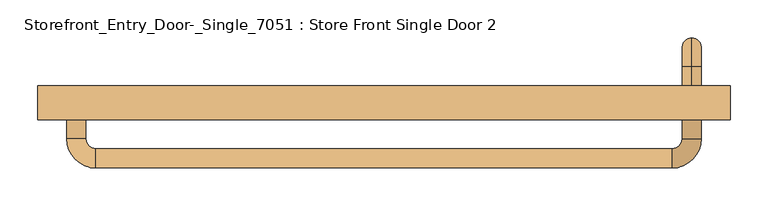
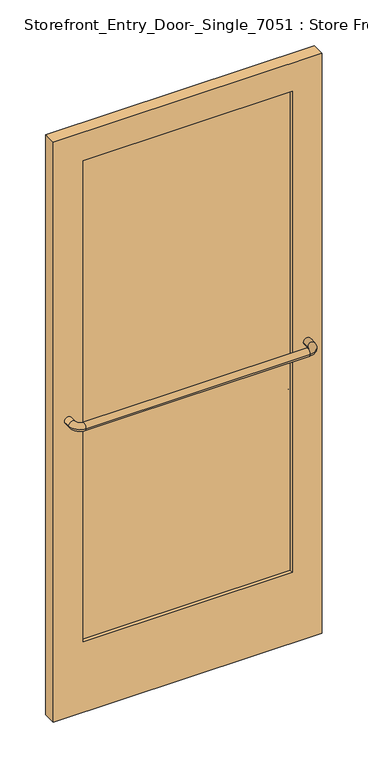
"""IFC4 building model written with IfcOpenShell, lengths in millimetres: door geometry, Storefront_Entry_Door-_Single_7051 : Store Front Single Door 2."""

from ifc_helpers import new_model, si_unit, point, frame, origin, place, context, project, spatial, polyline, circle_curve, ellipse_curve, trimmed, outline, extrude, source, transform, mapped, element, save
from ifc_brep_helpers import plane_surface, cylinder_surface, revolved_surface, advanced_brep


def storefront_entry_door_single_7051_store_front_single_door_2_9c77ce60(model_context):
    return source(origin(), model_context, "Body", "SolidModel", [
        advanced_brep(
        [(406.4, 50.8, 1054.1), (406.4, 50.8, 1079.5), (406.4, 76.2, 1054.1), (406.4, 76.2, 1079.5), (406.4, 114.3, 1041.4), (406.4, 88.9, 1041.4), (406.4, 88.9, 863.6), (406.4, 114.3, 863.6), (406.4, 76.2, 825.5), (406.4, 76.2, 850.9), (406.4, 50.8, 850.9), (406.4, 50.8, 825.5)],
        [
            (0, 1, circle_curve(frame((406.4, 50.8, 1066.8), z_axis=(0.0, -1.0, 0.0), x_axis=(0.0, 0.0, 1.0)), 12.7)),
            (1, 0, circle_curve(frame((406.4, 50.8, 1066.8), z_axis=(0.0, -1.0, 0.0), x_axis=(0.0, 0.0, 1.0)), 12.7)),
            (0, 2),
            (2, 3, circle_curve(frame((406.4, 76.2, 1066.8), z_axis=(0.0, -1.0, 0.0), x_axis=(0.0, 0.0, 1.0)), 12.7)),
            (3, 1),
            (3, 2, circle_curve(frame((406.4, 76.2, 1066.8), z_axis=(0.0, -1.0, 0.0), x_axis=(0.0, 0.0, 1.0)), 12.7)),
            (4, 3, circle_curve(frame((406.4, 76.2, 1041.4), z_axis=(1.0, 0.0, 0.0), x_axis=(0.0, 0.0, 1.0)), 38.1)),
            (2, 5, circle_curve(frame((406.4, 76.2, 1041.4), z_axis=(-1.0, 0.0, 0.0), x_axis=(0.0, 0.0, 1.0)), 12.7)),
            (5, 4, circle_curve(frame((406.4, 101.6, 1041.4), z_axis=(0.0, 0.0, 1.0), x_axis=(0.0, 1.0, 0.0)), 12.7)),
            (4, 5, circle_curve(frame((406.4, 101.6, 1041.4), z_axis=(0.0, 0.0, 1.0), x_axis=(0.0, 1.0, 0.0)), 12.7)),
            (5, 6),
            (6, 7, circle_curve(frame((406.4, 101.6, 863.6), z_axis=(0.0, 0.0, 1.0), x_axis=(0.0, 1.0, 0.0)), 12.7)),
            (7, 4),
            (7, 6, circle_curve(frame((406.4, 101.6, 863.6), z_axis=(0.0, 0.0, 1.0), x_axis=(0.0, 1.0, 0.0)), 12.7)),
            (8, 7, circle_curve(frame((406.4, 76.2, 863.6), z_axis=(1.0, 0.0, 0.0), x_axis=(0.0, 1.0, 0.0)), 38.1)),
            (6, 9, circle_curve(frame((406.4, 76.2, 863.6), z_axis=(-1.0, 0.0, 0.0), x_axis=(0.0, 1.0, 0.0)), 12.7)),
            (9, 8, circle_curve(frame((406.4, 76.2, 838.2), z_axis=(0.0, 1.0, 0.0), x_axis=(0.0, 0.0, -1.0)), 12.7)),
            (8, 9, circle_curve(frame((406.4, 76.2, 838.2), z_axis=(0.0, 1.0, 0.0), x_axis=(0.0, 0.0, -1.0)), 12.7)),
            (10, 11, circle_curve(frame((406.4, 50.8, 838.2), z_axis=(0.0, -1.0, 0.0), x_axis=(0.0, 0.0, -1.0)), 12.7)),
            (11, 10, circle_curve(frame((406.4, 50.8, 838.2), z_axis=(0.0, -1.0, 0.0), x_axis=(0.0, 0.0, -1.0)), 12.7)),
            (9, 10),
            (11, 8),
        ],
        [
            plane_surface(frame((406.4, 50.8, 1066.8), z_axis=(0.0, -1.0, 0.0), x_axis=(1.0, 0.0, 0.0))),
            cylinder_surface(frame((406.4, 50.8, 1066.8), z_axis=(0.0, -1.0, 0.0), x_axis=(0.0, 0.0, 1.0)), 12.7),
            revolved_surface(trimmed(ellipse_curve(frame((406.4, 76.2, 1066.8), z_axis=(0.0, -1.0, 0.0), x_axis=(0.0, 0.0, 1.0)), 12.7, 12.7), [point((406.4, 76.2, 1054.1))], [point((406.4, 76.2, 1079.5))], True, "CARTESIAN"), (406.4, 76.2, 1041.4), (-1.0, 0.0, 0.0)),
            revolved_surface(trimmed(ellipse_curve(frame((406.4, 76.2, 1066.8), z_axis=(0.0, -1.0, 0.0), x_axis=(0.0, 0.0, 1.0)), 12.7, 12.7), [point((406.4, 76.2, 1079.5))], [point((406.4, 76.2, 1054.1))], True, "CARTESIAN"), (406.4, 76.2, 1041.4), (-1.0, 0.0, 0.0)),
            cylinder_surface(frame((406.4, 101.6, 1041.4), z_axis=(0.0, 0.0, 1.0), x_axis=(0.0, 1.0, 0.0)), 12.7),
            revolved_surface(trimmed(ellipse_curve(frame((406.4, 101.6, 863.6), z_axis=(0.0, 0.0, 1.0), x_axis=(0.0, 1.0, 0.0)), 12.7, 12.7), [point((406.4, 88.9, 863.6))], [point((406.4, 114.3, 863.6))], True, "CARTESIAN"), (406.4, 76.2, 863.6), (-1.0, 0.0, 0.0)),
            revolved_surface(trimmed(ellipse_curve(frame((406.4, 101.6, 863.6), z_axis=(0.0, 0.0, 1.0), x_axis=(0.0, 1.0, 0.0)), 12.7, 12.7), [point((406.4, 114.3, 863.6))], [point((406.4, 88.9, 863.6))], True, "CARTESIAN"), (406.4, 76.2, 863.6), (-1.0, 0.0, 0.0)),
            plane_surface(frame((406.4, 50.8, 838.2), z_axis=(0.0, -1.0, 0.0), x_axis=(1.0, 0.0, 0.0))),
            cylinder_surface(frame((406.4, 76.2, 838.2), z_axis=(0.0, 1.0, 0.0), x_axis=(0.0, 0.0, -1.0)), 12.7),
        ],
        [
            (0, [[1, 2]]),
            (1, [[-1, 3, 4, 5]]),
            (1, [[-2, -5, 6, -3]]),
            (2, [[7, -4, 8, 9]]),
            (3, [[-8, -6, -7, 10]]),
            (4, [[-9, 11, 12, 13]]),
            (4, [[-10, -13, 14, -11]]),
            (5, [[15, -12, 16, 17]]),
            (6, [[-16, -14, -15, 18]]),
            (7, [[19, 20]]),
            (8, [[-17, 21, -20, 22]]),
            (8, [[-18, -22, -19, -21]]),
        ],
    ),
        advanced_brep(
        [(393.7, 6.35, 1066.8), (419.1, 6.35, 1066.8), (393.7, -19.05, 1066.8), (419.1, -19.05, 1066.8), (381.0, -57.15, 1066.8), (381.0, -31.75, 1066.8), (-381.0, -31.75, 1066.8), (-381.0, -57.15, 1066.8), (-419.1, -19.05, 1066.8), (-393.7, -19.05, 1066.8), (-393.7, 6.35, 1066.8), (-419.1, 6.35, 1066.8)],
        [
            (0, 1, circle_curve(frame((406.4, 6.35, 1066.8), z_axis=(0.0, 1.0, 0.0), x_axis=(1.0, 0.0, 0.0)), 12.7)),
            (1, 0, circle_curve(frame((406.4, 6.35, 1066.8), z_axis=(0.0, 1.0, 0.0), x_axis=(1.0, 0.0, 0.0)), 12.7)),
            (0, 2),
            (2, 3, circle_curve(frame((406.4, -19.05, 1066.8), z_axis=(0.0, 1.0, 0.0), x_axis=(1.0, 0.0, 0.0)), 12.7)),
            (3, 1),
            (3, 2, circle_curve(frame((406.4, -19.05, 1066.8), z_axis=(0.0, 1.0, 0.0), x_axis=(1.0, 0.0, 0.0)), 12.7)),
            (4, 3, circle_curve(frame((381.0, -19.05, 1066.8), z_axis=(0.0, 0.0, 1.0), x_axis=(1.0, 0.0, 0.0)), 38.1)),
            (2, 5, circle_curve(frame((381.0, -19.05, 1066.8), z_axis=(0.0, 0.0, -1.0), x_axis=(1.0, 0.0, 0.0)), 12.7)),
            (5, 4, circle_curve(frame((381.0, -44.45, 1066.8), z_axis=(1.0, 0.0, 0.0), x_axis=(0.0, -1.0, 0.0)), 12.7)),
            (4, 5, circle_curve(frame((381.0, -44.45, 1066.8), z_axis=(1.0, 0.0, 0.0), x_axis=(0.0, -1.0, 0.0)), 12.7)),
            (5, 6),
            (6, 7, circle_curve(frame((-381.0, -44.45, 1066.8), z_axis=(1.0, 0.0, 0.0), x_axis=(0.0, -1.0, 0.0)), 12.7)),
            (7, 4),
            (7, 6, circle_curve(frame((-381.0, -44.45, 1066.8), z_axis=(1.0, 0.0, 0.0), x_axis=(0.0, -1.0, 0.0)), 12.7)),
            (8, 7, circle_curve(frame((-381.0, -19.05, 1066.8), z_axis=(0.0, 0.0, 1.0), x_axis=(0.0, -1.0, 0.0)), 38.1)),
            (6, 9, circle_curve(frame((-381.0, -19.05, 1066.8), z_axis=(0.0, 0.0, -1.0), x_axis=(0.0, -1.0, 0.0)), 12.7)),
            (9, 8, circle_curve(frame((-406.4, -19.05, 1066.8), z_axis=(0.0, -1.0, 0.0), x_axis=(-1.0, 0.0, 0.0)), 12.7)),
            (8, 9, circle_curve(frame((-406.4, -19.05, 1066.8), z_axis=(0.0, -1.0, 0.0), x_axis=(-1.0, 0.0, 0.0)), 12.7)),
            (10, 11, circle_curve(frame((-406.4, 6.35, 1066.8), z_axis=(0.0, 1.0, 0.0), x_axis=(-1.0, 0.0, 0.0)), 12.7)),
            (11, 10, circle_curve(frame((-406.4, 6.35, 1066.8), z_axis=(0.0, 1.0, 0.0), x_axis=(-1.0, 0.0, 0.0)), 12.7)),
            (9, 10),
            (11, 8),
        ],
        [
            plane_surface(frame((406.4, 6.35, 1066.8), z_axis=(0.0, 1.0, 0.0), x_axis=(0.0, 0.0, 1.0))),
            cylinder_surface(frame((406.4, 6.35, 1066.8), z_axis=(0.0, 1.0, 0.0), x_axis=(1.0, 0.0, 0.0)), 12.7),
            revolved_surface(trimmed(ellipse_curve(frame((406.4, -19.05, 1066.8), z_axis=(0.0, 1.0, 0.0), x_axis=(1.0, 0.0, 0.0)), 12.7, 12.7), [point((393.7, -19.05, 1066.8))], [point((419.1, -19.05, 1066.8))], True, "CARTESIAN"), (381.0, -19.05, 1066.8), (0.0, 0.0, -1.0)),
            revolved_surface(trimmed(ellipse_curve(frame((406.4, -19.05, 1066.8), z_axis=(0.0, 1.0, 0.0), x_axis=(1.0, 0.0, 0.0)), 12.7, 12.7), [point((419.1, -19.05, 1066.8))], [point((393.7, -19.05, 1066.8))], True, "CARTESIAN"), (381.0, -19.05, 1066.8), (0.0, 0.0, -1.0)),
            cylinder_surface(frame((381.0, -44.45, 1066.8), z_axis=(1.0, 0.0, 0.0), x_axis=(0.0, -1.0, 0.0)), 12.7),
            revolved_surface(trimmed(ellipse_curve(frame((-381.0, -44.45, 1066.8), z_axis=(1.0, 0.0, 0.0), x_axis=(0.0, -1.0, 0.0)), 12.7, 12.7), [point((-381.0, -31.75, 1066.8))], [point((-381.0, -57.15, 1066.8))], True, "CARTESIAN"), (-381.0, -19.05, 1066.8), (0.0, 0.0, -1.0)),
            revolved_surface(trimmed(ellipse_curve(frame((-381.0, -44.45, 1066.8), z_axis=(1.0, 0.0, 0.0), x_axis=(0.0, -1.0, 0.0)), 12.7, 12.7), [point((-381.0, -57.15, 1066.8))], [point((-381.0, -31.75, 1066.8))], True, "CARTESIAN"), (-381.0, -19.05, 1066.8), (0.0, 0.0, -1.0)),
            plane_surface(frame((-406.4, 6.35, 1066.8), z_axis=(0.0, 1.0, 0.0), x_axis=(0.0, 0.0, 1.0))),
            cylinder_surface(frame((-406.4, -19.05, 1066.8), z_axis=(0.0, -1.0, 0.0), x_axis=(-1.0, 0.0, 0.0)), 12.7),
        ],
        [
            (0, [[1, 2]]),
            (1, [[-1, 3, 4, 5]]),
            (1, [[-2, -5, 6, -3]]),
            (2, [[7, -4, 8, 9]]),
            (3, [[-8, -6, -7, 10]]),
            (4, [[-9, 11, 12, 13]]),
            (4, [[-10, -13, 14, -11]]),
            (5, [[15, -12, 16, 17]]),
            (6, [[-16, -14, -15, 18]]),
            (7, [[19, 20]]),
            (8, [[-17, 21, -20, 22]]),
            (8, [[-18, -22, -19, -21]]),
        ],
    ),
        extrude(outline(polyline([(355.6, 19.05), (-355.6, 19.05), (-355.6, 38.1), (355.6, 38.1), (355.6, 19.05)])), frame((0.0, 0.0, 254.0), z_axis=(0.0, 0.0, 1.0), x_axis=(1.0, 0.0, 0.0)), (0.0, 0.0, 1.0), 1727.2),
        extrude(outline(polyline([(2082.8, 457.2), (2082.8, -457.2), (0.0, -457.2), (0.0, 457.2), (2082.8, 457.2)]), holes=[polyline([(1981.2, -355.6), (1981.2, 355.6), (254.0, 355.6), (254.0, -355.6), (1981.2, -355.6)])]), frame((0.0, 6.35, 0.0), z_axis=(0.0, 1.0, 0.0), x_axis=(0.0, 0.0, 1.0)), (0.0, 0.0, 1.0), 44.45),
    ])


if __name__ == "__main__":
    model = new_model("IFC4")
    model_context = context("Model", 3, world=origin())
    ifc_project = project(units=[si_unit("LENGTHUNIT", "METRE", prefix="MILLI")], contexts=[model_context])
    site = spatial("IfcSite", under=ifc_project)
    building = spatial("IfcBuilding", under=site)
    placement = place(None, origin())
    storefront_entry_door_single_7051_store_front_single_door_2_shape = storefront_entry_door_single_7051_store_front_single_door_2_9c77ce60(model_context)
    element("IfcDoor", 1, ObjectType="Storefront_Entry_Door-_Single_7051 : Store Front Single Door 2", at=placement, inside=building, context=model_context, shape_type="MappedRepresentation", body=[
        mapped(storefront_entry_door_single_7051_store_front_single_door_2_shape, transform((0.0, 0.0, 0.0), x_axis=(1.0, 0.0, 0.0), y_axis=(0.0, 1.0, 0.0), z_axis=(0.0, 0.0, 1.0))),
    ])
    save(model, "model.ifc")

# Revit data of these elements
# Type "Storefront_Entry_Door-_Single_7051 : Store Front Single Door 2"
#   Type Mark = "01"
#   Assembly Code = "B2030110"
#   Analytic Construction = "<None>"
#   Top Rail = 0' - 4"
#   Side Rail = 0' - 4"
#   Reporting Width [instance default] = 4' - 2"
#   Rail Height AFF = 3' - 6"
#   Offset = 0' - 2"
#   Door Width [instance default] = 4' - 2"
#   Bottom Rail Width = 0' - 10"
#   Material = ALUM. STOREFRONT
#   Glazing Material = INSULATED GLAZING - <0.32 U-VALUE & <0.23 SHGC
#   Function = (empty or 0)
# Element 1 (IfcDoor, "Storefront_Entry_Door-_Single_7051 : Store Front Single Door 2")
#   Reporting Width = 3' - 0"
#   Door Width = 3' - 0"
#   Materials on its faces: "ALUM. STOREFRONT", "INSULATED GLAZING - <0.32 U-VALUE & <0.23 SHGC"
# Materials
#   "ALUM. STOREFRONT": class "Generic", colour RGB 92 104 51, transparency 0, Cost = 0
#   "INSULATED GLAZING - <0.32 U-VALUE & <0.23 SHGC": class "Glass", colour RGB 236 240 239, transparency 0.85, Description = "Soda Lime Glass", Cost = 0
